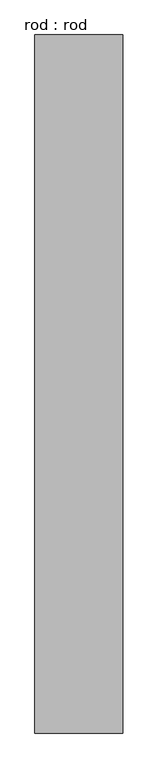
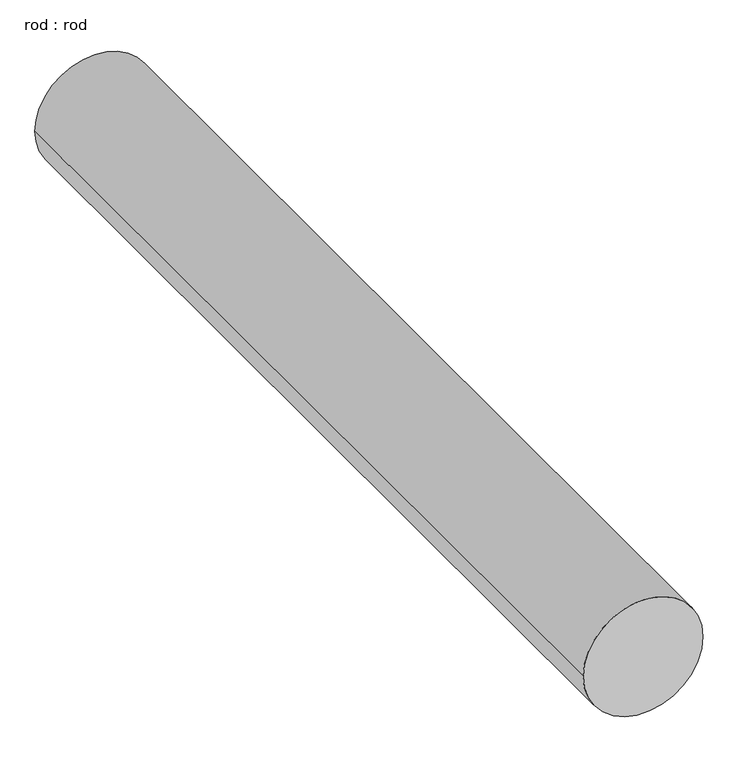
"""IFC4 building model written with IfcOpenShell, lengths in millimetres: proxy geometry, rod : rod."""

from ifc_helpers import new_model, si_unit, point, frame, frame_2d, origin, place, context, project, spatial, circle_curve, trimmed, segment, composite_curve, outline, extrude, source, transform, mapped, element, save


def rod_rod_ac689943(model_context):
    return source(origin(), model_context, "Body", "SweptSolid", [
        extrude(outline(composite_curve([segment(trimmed(circle_curve(frame_2d((0.0108462, 0.0)), 200.0), [point((0.0108462, 200.0))], [point((0.0108462, -200.0))], False, "CARTESIAN"), True, "CONTINUOUS"), segment(trimmed(circle_curve(frame_2d((0.0108462, 0.0)), 200.0), [point((0.0108462, -200.0))], [point((0.0108462, 200.0))], False, "CARTESIAN"), True, "CONTINUOUS")], self_intersect=False)), frame((0.0, 2507.0143296, 0.0), z_axis=(0.0, 1.0, 0.0), x_axis=(0.0, 0.0, 1.0)), (0.0, 0.0, 1.0), 3171.4285714),
    ])


if __name__ == "__main__":
    model = new_model("IFC4")
    model_context = context("Model", 3, world=origin())
    ifc_project = project(units=[si_unit("LENGTHUNIT", "METRE", prefix="MILLI")], contexts=[model_context])
    site = spatial("IfcSite", under=ifc_project)
    building = spatial("IfcBuilding", under=site)
    placement = place(None, origin())
    rod_rod_shape = rod_rod_ac689943(model_context)
    element("IfcBuildingElementProxy", 1, Name="rod : rod", ObjectType="rod : rod", at=placement, inside=building, context=model_context, shape_type="MappedRepresentation", body=[
        mapped(rod_rod_shape, transform((0.0, 0.0, 0.0), x_axis=(1.0, 0.0, 0.0), y_axis=(0.0, 1.0, 0.0), z_axis=(0.0, 0.0, 1.0))),
    ])
    save(model, "model.ifc")

# Revit data of these elements
# Type "rod : rod"
#   Default Elevation = 0
